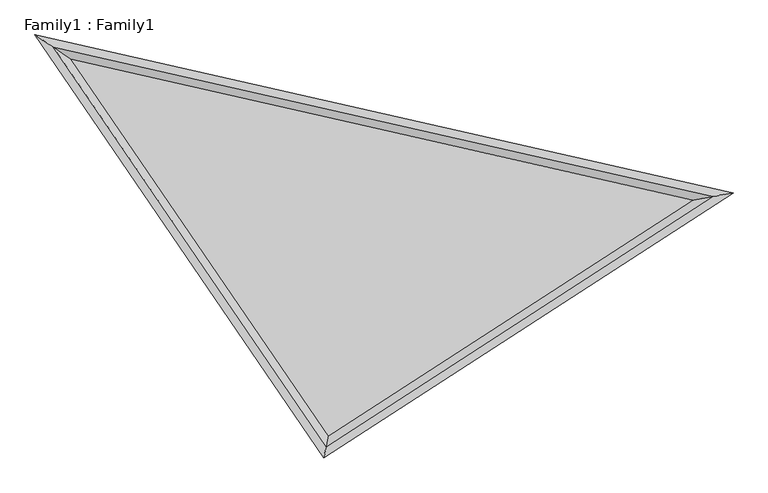
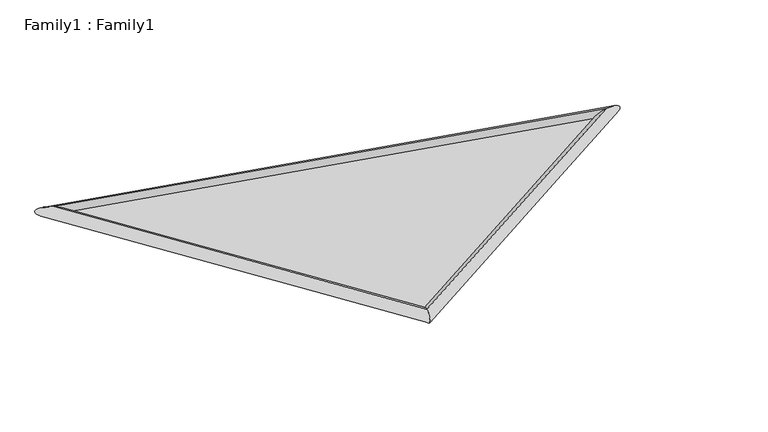
"""IFC4 building model written with IfcOpenShell, lengths in millimetres: proxy geometry, Family1 : Family1."""

from ifc_helpers import new_model, si_unit, frame, origin, origin_with_axes, place, context, project, spatial, polyline, ellipse_curve, outline, extrude, source, transform, mapped, element, save
from ifc_brep_helpers import cylinder_surface, advanced_brep


def family1_family1_9af2231e(model_context):
    return source(origin(), model_context, "Body", "SolidModel", [
        extrude(outline(polyline([(457.9326687, -2199.394534), (-2894.3870171, 2709.6937681), (5203.3767994, 873.6419708), (457.9326687, -2199.394534)])), origin_with_axes(), (0.0, 0.0, 1.0), 34.1328789),
        advanced_brep(
        [(457.9326687, -2199.394534, 100.0), (457.9326687, -2199.394534, -100.0), (-2894.3870171, 2709.6937681, -100.0), (-2894.3870171, 2709.6937681, 100.0), (5203.3767994, 873.6419708, -100.0), (5203.3767994, 873.6419708, 100.0)],
        [
            (0, 1, ellipse_curve(frame((457.9326687, -2199.394534, 0.0), z_axis=(-0.980365122758794, 0.19719083669921064, 0.0), x_axis=(-0.19719083669921056, -0.9803651227587941, 0.0)), 139.7220683, 100.0)),
            (1, 2),
            (2, 3, ellipse_curve(frame((-2894.3870171, 2709.6937681, 0.0), z_axis=(-0.562419695800743, -0.8268519128449784, 0.0), x_axis=(0.8268519128449783, -0.562419695800743, 0.0)), 273.4769585, 100.0)),
            (3, 0),
            (1, 0, ellipse_curve(frame((457.9326687, -2199.394534, 0.0), z_axis=(-0.980365122758794, 0.19719083669921064, 0.0), x_axis=(-0.19719083669921056, -0.9803651227587941, 0.0)), 139.7220683, 100.0)),
            (3, 2, ellipse_curve(frame((-2894.3870171, 2709.6937681, 0.0), z_axis=(-0.562419695800743, -0.8268519128449784, 0.0), x_axis=(0.8268519128449783, -0.562419695800743, 0.0)), 273.4769585, 100.0)),
            (2, 4),
            (4, 5, ellipse_curve(frame((5203.3767994, 873.6419708, 0.0), z_axis=(-0.1749468425795881, 0.9845778802468766, 0.0), x_axis=(-0.9845778802468765, -0.17494684257958815, 0.0)), 257.5135809, 100.0)),
            (5, 3),
            (5, 4, ellipse_curve(frame((5203.3767994, 873.6419708, 0.0), z_axis=(-0.1749468425795881, 0.9845778802468766, 0.0), x_axis=(-0.9845778802468765, -0.17494684257958815, 0.0)), 257.5135809, 100.0)),
            (4, 1),
            (0, 5),
        ],
        [
            cylinder_surface(frame((457.9326687, -2199.394534, 0.0), z_axis=(0.56393544145874, -0.8258188771557211, 0.0), x_axis=(-0.8258188771557211, -0.56393544145874, 0.0)), 100.0),
            cylinder_surface(frame((-2894.3870171, 2709.6937681, 0.0), z_axis=(-0.9752459218014271, 0.22112302460323927, 0.0), x_axis=(0.22112302460323927, 0.9752459218014271, 0.0)), 100.0),
            cylinder_surface(frame((5203.3767994, 873.6419708, 0.0), z_axis=(0.8393720451824259, 0.5435573288681439, 0.0), x_axis=(0.5435573288681439, -0.8393720451824259, 0.0)), 100.0),
        ],
        [
            (0, [[1, 2, 3, 4]]),
            (0, [[5, -4, 6, -2]]),
            (1, [[-3, 7, 8, 9]]),
            (1, [[-6, -9, 10, -7]]),
            (2, [[-8, 11, -1, 12]]),
            (2, [[-10, -12, -5, -11]]),
        ],
    ),
    ])


if __name__ == "__main__":
    model = new_model("IFC4")
    model_context = context("Model", 3, world=origin())
    ifc_project = project(units=[si_unit("LENGTHUNIT", "METRE", prefix="MILLI")], contexts=[model_context])
    site = spatial("IfcSite", under=ifc_project)
    building = spatial("IfcBuilding", under=site)
    placement = place(None, origin())
    family1_family1_shape = family1_family1_9af2231e(model_context)
    element("IfcBuildingElementProxy", 1, Name="Family1 : Family1", ObjectType="Family1 : Family1", at=placement, inside=building, context=model_context, shape_type="MappedRepresentation", body=[
        mapped(family1_family1_shape, transform((0.0, 0.0, 0.0), x_axis=(1.0, 0.0, 0.0), y_axis=(0.0, 1.0, 0.0), z_axis=(0.0, 0.0, 1.0))),
    ])
    save(model, "model.ifc")

# Revit data of these elements
# Type "Family1 : Family1"
#   Default Elevation = 0
# Element 1 (IfcBuildingElementProxy, "Family1 : Family1")
#   Materials on its faces: "Glass"
# Materials
#   "Glass": class "Glass", colour RGB 0 128 192, transparency 0.9, Description = "Soda Lime Glass", Cost = 0
